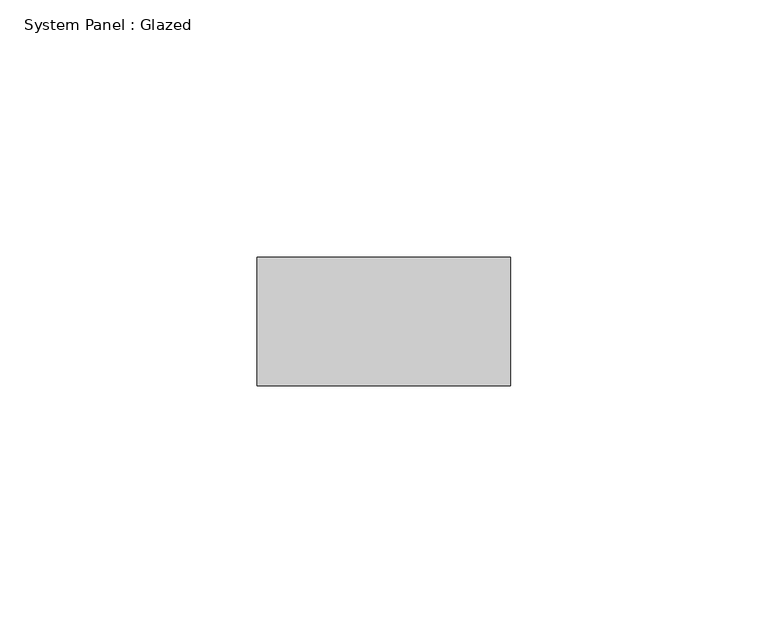
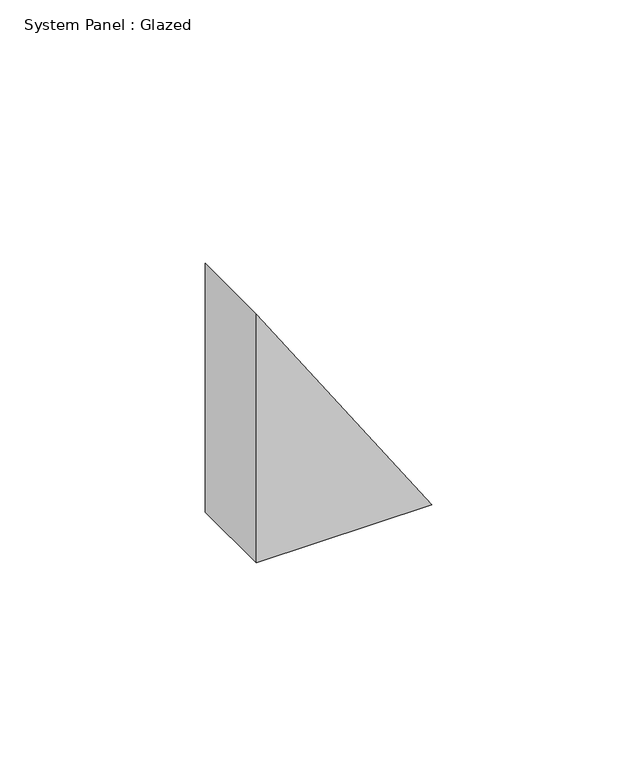
"""IFC4 building model written with IfcOpenShell, lengths in millimetres: plate geometry, System Panel : Glazed."""

import ifcopenshell
import ifcopenshell.guid

model = None  # the IFC model being written
_history = None  # IfcOwnerHistory: only IFC2X3 demands one
_inside = {}  # id of a spatial element -> (the spatial element, [elements in it])
_under = {}  # id of a project, library or spatial element -> (it, [spatial elements below it])
_declared = {}  # id of a project -> (the project, [libraries it declares])
_typed = {}  # id of a type object -> (the type object, [elements of that type])
_made_of = {}  # id of a material, layer set ... -> (it, [elements and type objects made of it])


def new_model(schema):
    """Start an empty IFC model of exactly this schema.

    Asked for "IFC4X3", IfcOpenShell would pick the latest addendum, in which some entities
    have other attributes; the version numbers below select the first issue.
    IFC2X3 requires an IfcOwnerHistory on every rooted entity: one is made here for all.
    """
    global model, _history
    if schema == "IFC4X3":
        model = ifcopenshell.file(schema_version=(4, 3, 0, 0))
    else:
        model = ifcopenshell.file(schema=schema)
    _inside.clear()
    _under.clear()
    _declared.clear()
    _typed.clear()
    _made_of.clear()
    _history = None
    if model.schema == "IFC2X3":
        org = make("IfcOrganization", Name="unknown")
        user = make(
            "IfcPersonAndOrganization",
            ThePerson=make("IfcPerson", FamilyName="unknown"),
            TheOrganization=org,
        )
        app = make(
            "IfcApplication",
            ApplicationDeveloper=org,
            Version="unknown",
            ApplicationFullName="unknown",
            ApplicationIdentifier="unknown",
        )
        _history = make(
            "IfcOwnerHistory",
            OwningUser=user,
            OwningApplication=app,
            ChangeAction="ADDED",
            CreationDate=0,
        )
    return model


def make(cls, **values):
    """One entity of the class cls with the attributes given. An attribute that is None is left unset."""
    return model.create_entity(
        cls, **{name: value for name, value in values.items() if value is not None}
    )


def rooted(cls, **values):
    """An entity with a GlobalId (a new one), such as an element, a storey or a relation."""
    return make(cls, GlobalId=ifcopenshell.guid.new(), OwnerHistory=_history, **values)


def si_unit(unit_type, name, prefix=None):
    """IfcSIUnit, for example si_unit("LENGTHUNIT", "METRE", prefix="MILLI")."""
    return make("IfcSIUnit", UnitType=unit_type, Prefix=prefix, Name=name)


def assignment(units):
    """IfcUnitAssignment: the units of a project."""
    return None if units is None else make("IfcUnitAssignment", Units=units)


def point(xyz):
    """IfcCartesianPoint."""
    return None if xyz is None else make("IfcCartesianPoint", Coordinates=xyz)


def direction(xyz):
    """IfcDirection."""
    return None if xyz is None else make("IfcDirection", DirectionRatios=xyz)


def frame(location, z_axis=None, x_axis=None):
    """IfcAxis2Placement3D, a coordinate frame: its origin and axes. An axis left out is left unset."""
    return make(
        "IfcAxis2Placement3D",
        Location=point(location),
        Axis=direction(z_axis),
        RefDirection=direction(x_axis),
    )


def origin():
    """The frame at (0, 0, 0) with its axes left unset."""
    return frame((0.0, 0.0, 0.0))


def place(relative_to, where):
    """IfcLocalPlacement: puts the frame where relative to a parent placement (None: the world)."""
    return make(
        "IfcLocalPlacement", PlacementRelTo=relative_to, RelativePlacement=where
    )


def context(
    kind, dimensions, precision=None, world=None, true_north=None, identifier=None
):
    """IfcGeometricRepresentationContext, for example the 3D "Model" context."""
    return make(
        "IfcGeometricRepresentationContext",
        ContextIdentifier=identifier,
        ContextType=kind,
        CoordinateSpaceDimension=dimensions,
        Precision=precision,
        WorldCoordinateSystem=world,
        TrueNorth=true_north,
    )


def project(units=None, contexts=None):
    """IfcProject with its units and contexts."""
    return rooted(
        "IfcProject",
        Name="project",
        RepresentationContexts=contexts,
        UnitsInContext=assignment(units),
    )


def spatial(cls, under=None, at=None, **own):
    """A site, building, storey or space (cls), placed at a placement, below another one or the project."""
    s = rooted(cls, ObjectPlacement=at, **own)
    if under is not None:
        _under.setdefault(under.id(), (under, []))[1].append(s)
    return s


def polyline(points):
    """IfcPolyline through the points."""
    return make("IfcPolyline", Points=[point(p) for p in points])


def outline(outer, holes=None, kind="AREA"):
    """IfcArbitraryClosedProfileDef: a profile drawn as a closed curve; with holes, ...WithVoids."""
    if holes is None:
        return make("IfcArbitraryClosedProfileDef", ProfileType=kind, OuterCurve=outer)
    return make(
        "IfcArbitraryProfileDefWithVoids",
        ProfileType=kind,
        OuterCurve=outer,
        InnerCurves=holes,
    )


def extrude(swept, where, along, depth):
    """IfcExtrudedAreaSolid: the profile swept, set in the frame where, extruded along a direction by depth."""
    return make(
        "IfcExtrudedAreaSolid",
        SweptArea=swept,
        Position=where,
        ExtrudedDirection=direction(along),
        Depth=depth,
    )


def shape(context_of_items, identifier, shape_type, items):
    """IfcShapeRepresentation: the items that make up one representation, for example the "Body"."""
    return make(
        "IfcShapeRepresentation",
        ContextOfItems=context_of_items,
        RepresentationIdentifier=identifier,
        RepresentationType=shape_type,
        Items=items,
    )


def source(mapping_origin, context_of_items, identifier, shape_type, items):
    """IfcRepresentationMap: a shape defined once, which mapped items show again and again."""
    return make(
        "IfcRepresentationMap",
        MappingOrigin=mapping_origin,
        MappedRepresentation=shape(context_of_items, identifier, shape_type, items),
    )


def transform(
    local_origin,
    x_axis=None,
    y_axis=None,
    z_axis=None,
    scale=None,
    scale2=None,
    scale3=None,
    uniform=True,
):
    """IfcCartesianTransformationOperator3D, or its non-uniform kind. x_axis, y_axis, z_axis: its Axis1, 2, 3."""
    if uniform:
        return make(
            "IfcCartesianTransformationOperator3D",
            Axis1=direction(x_axis),
            Axis2=direction(y_axis),
            LocalOrigin=point(local_origin),
            Scale=scale,
            Axis3=direction(z_axis),
        )
    return make(
        "IfcCartesianTransformationOperator3DnonUniform",
        Axis1=direction(x_axis),
        Axis2=direction(y_axis),
        LocalOrigin=point(local_origin),
        Scale=scale,
        Axis3=direction(z_axis),
        Scale2=scale2,
        Scale3=scale3,
    )


def mapped(mapping_source, mapping_target):
    """IfcMappedItem: shows the shape of a source again, moved by a transform."""
    return make(
        "IfcMappedItem", MappingSource=mapping_source, MappingTarget=mapping_target
    )


def made_of(thing, what):
    """Note that an element or type object is made of a material, layer set ...; save() writes the relation."""
    if what is not None:
        _made_of.setdefault(what.id(), (what, []))[1].append(thing)
    return thing


def element(
    cls,
    number,
    at=None,
    inside=None,
    cuts=None,
    type_object=None,
    material=None,
    context=None,
    identifier="Body",
    shape_type=None,
    held_by="IfcProductDefinitionShape",
    body=None,
    shapes=None,
    **own,
):
    """One element of the class cls, such as IfcWall. Its Tag is "e" and its number.

    at: its placement. inside: the storey or other place that contains it. cuts: it is an
    opening in that element (IfcRelVoidsElement). A single representation is given by context,
    identifier, shape_type and body (its items); several are given by shapes. held_by: the class
    of the entity that holds the representations. save() writes the other relations.
    """
    e = rooted(cls, Tag="e%d" % number, ObjectPlacement=at, **own)
    if body is not None:
        shapes = [shape(context, identifier, shape_type, body)]
    if shapes is not None:
        e.Representation = make(held_by, Representations=shapes)
    if inside is not None:
        _inside.setdefault(inside.id(), (inside, []))[1].append(e)
    if cuts is not None:
        rooted(
            "IfcRelVoidsElement", RelatingBuildingElement=cuts, RelatedOpeningElement=e
        )
    if type_object is not None:
        _typed.setdefault(type_object.id(), (type_object, []))[1].append(e)
    return made_of(e, material)


def aggregate(whole, parts):
    """IfcRelAggregates: a whole, such as a stair, and the parts it consists of."""
    return rooted("IfcRelAggregates", RelatingObject=whole, RelatedObjects=parts)


def save(model, path):
    """Write the relations noted so far, then the file.

    IfcRelAggregates (storeys below a building ...), IfcRelContainedInSpatialStructure (elements
    in a storey), IfcRelDefinesByType, IfcRelAssociatesMaterial and IfcRelDeclares: one each for
    every whole, place, type object, material and project.
    """
    for whole, parts in _under.values():
        aggregate(whole, parts)
    for where, things in _inside.values():
        rooted(
            "IfcRelContainedInSpatialStructure",
            RelatedElements=things,
            RelatingStructure=where,
        )
    for kind, things in _typed.values():
        rooted("IfcRelDefinesByType", RelatedObjects=things, RelatingType=kind)
    for what, things in _made_of.values():
        rooted("IfcRelAssociatesMaterial", RelatedObjects=things, RelatingMaterial=what)
    for by, libraries in _declared.values():
        rooted("IfcRelDeclares", RelatingContext=by, RelatedDefinitions=libraries)
    model.write(path)


def system_panel_glazed_44b53722(model_context):
    return source(origin(), model_context, "Body", "SweptSolid", [
        extrude(outline(polyline([(0.0, -24.6975445), (0.0, 24.6975445), (74.0824486, -24.6975445), (0.0, -24.6975445)])), frame((0.0, 24.5, 0.0), z_axis=(0.0, 1.0, 0.0), x_axis=(0.0, 0.0, 1.0)), (0.0, 0.0, 1.0), 25.0),
    ])


if __name__ == "__main__":
    model = new_model("IFC4")
    model_context = context("Model", 3, world=origin())
    ifc_project = project(units=[si_unit("LENGTHUNIT", "METRE", prefix="MILLI")], contexts=[model_context])
    site = spatial("IfcSite", under=ifc_project)
    building = spatial("IfcBuilding", under=site)
    placement = place(None, origin())
    system_panel_glazed_shape = system_panel_glazed_44b53722(model_context)
    element("IfcPlate", 1, ObjectType="System Panel : Glazed", at=placement, inside=building, context=model_context, shape_type="MappedRepresentation", body=[
        mapped(system_panel_glazed_shape, transform((0.0, 0.0, 0.0), x_axis=(1.0, 0.0, 0.0), y_axis=(0.0, 1.0, 0.0), z_axis=(0.0, 0.0, 1.0))),
    ])
    save(model, "model.ifc")

# Revit data of these elements
# Type "System Panel : Glazed"
#   Keynote = "H11"
#   Construction Type Id = "GSP4R"
#   Analytic Construction = "1/8 in Pilkington single glazing"
#   Visual Light Transmittance = 0.9
#   Solar Heat Gain Coefficient = 0.86
#   Heat Transfer Coefficient (U) = 6.7069 W/(m²·K)
#   Define Thermal Properties by = 1
# Element 1 (IfcPlate, "System Panel : Glazed")
#   Materials on its faces: "Glass"
# Materials
#   "Glass": class "Glass", colour RGB 0 128 192, transparency 0.9, Description = "Soda Lime Glass", Cost = 0
